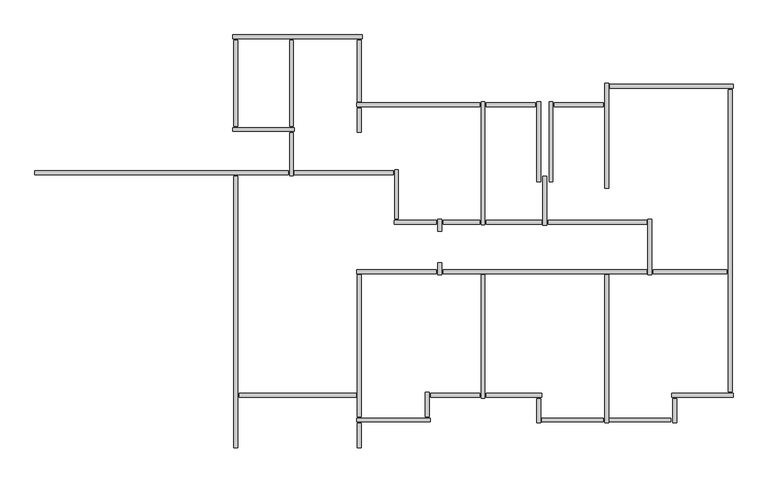
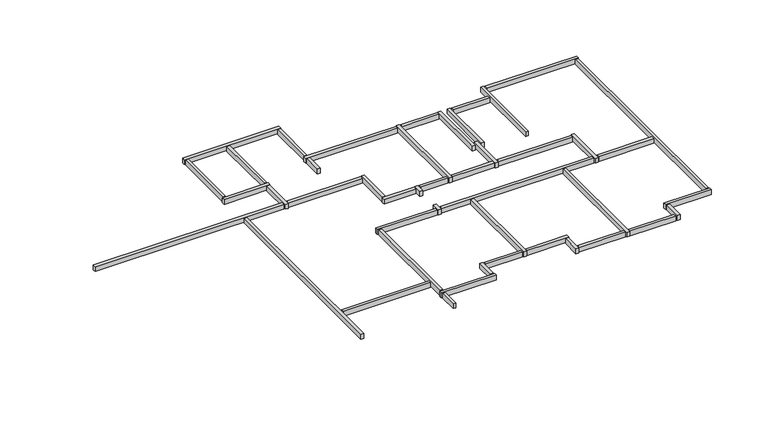
"""IFC4 building model written with IfcOpenShell, lengths in millimetres: beam geometry, Graute viga de respaldo12 : Graute viga de respaldo."""

from ifc_helpers import new_model, si_unit, frame, origin, place, context, project, spatial, polyline, outline, extrude, source, transform, mapped, element, save


def beam_e93206ce(model_context):
    return source(origin(), model_context, "Body", "SweptSolid", [
        extrude(outline(polyline([(-54994.9587292, 57408.4278788), (-54994.9587292, 57502.4278788), (-53804.9587292, 57502.4278788), (-53804.9587292, 57408.4278788), (-54994.9587292, 57408.4278788)])), frame((0.0, 0.0, 11632.9999999), z_axis=(0.0, 0.0, 1.0), x_axis=(1.0, 0.0, 0.0)), (0.0, 0.0, 1.0), 167.0),
        extrude(outline(polyline([(-56644.9587292, 57408.4278788), (-56644.9587292, 57502.4278788), (-55454.9587292, 57502.4278788), (-55454.9587292, 57408.4278788), (-56644.9587292, 57408.4278788)])), frame((0.0, 0.0, 11632.9999999), z_axis=(0.0, 0.0, 1.0), x_axis=(1.0, 0.0, 0.0)), (0.0, 0.0, 1.0), 167.0),
        extrude(outline(polyline([(-52594.9587292, 53358.4278788), (-52594.9587292, 53452.4278788), (-50804.9587292, 53452.4278788), (-50804.9587292, 53358.4278788), (-52594.9587292, 53358.4278788)])), frame((0.0, 0.0, 11632.9999999), z_axis=(0.0, 0.0, 1.0), x_axis=(1.0, 0.0, 0.0)), (0.0, 0.0, 1.0), 167.0),
        extrude(outline(polyline([(-57994.9587292, 50358.4278788), (-57994.9587292, 50452.4278788), (-56804.9587292, 50452.4278788), (-56804.9587292, 50358.4278788), (-57994.9587292, 50358.4278788)])), frame((0.0, 0.0, 11632.9999999), z_axis=(0.0, 0.0, 1.0), x_axis=(1.0, 0.0, 0.0)), (0.0, 0.0, 1.0), 167.0),
        extrude(outline(polyline([(-58121.9587292, 50475.4278788), (-58027.9587292, 50475.4278788), (-58027.9587292, 49885.4278788), (-58121.9587292, 49885.4278788), (-58121.9587292, 50475.4278788)])), frame((0.0, 0.0, 11632.9999999), z_axis=(0.0, 0.0, 1.0), x_axis=(1.0, 0.0, 0.0)), (0.0, 0.0, 1.0), 167.0),
        extrude(outline(polyline([(-59794.9587292, 49758.4278788), (-59794.9587292, 49852.4278788), (-58004.9587292, 49852.4278788), (-58004.9587292, 49758.4278788), (-59794.9587292, 49758.4278788)])), frame((0.0, 0.0, 11632.9999999), z_axis=(0.0, 0.0, 1.0), x_axis=(1.0, 0.0, 0.0)), (0.0, 0.0, 1.0), 167.0),
        extrude(outline(polyline([(-57727.9587292, 53335.4278788), (-57821.9587292, 53335.4278788), (-57821.9587292, 53625.4278788), (-57727.9587292, 53625.4278788), (-57727.9587292, 53335.4278788)])), frame((0.0, 0.0, 11632.9999999), z_axis=(0.0, 0.0, 1.0), x_axis=(1.0, 0.0, 0.0)), (0.0, 0.0, 1.0), 167.0),
        extrude(outline(polyline([(-55144.9587292, 54558.4278788), (-55144.9587292, 54652.4278788), (-52754.9587292, 54652.4278788), (-52754.9587292, 54558.4278788), (-55144.9587292, 54558.4278788)])), frame((0.0, 0.0, 11632.9999999), z_axis=(0.0, 0.0, 1.0), x_axis=(1.0, 0.0, 0.0)), (0.0, 0.0, 1.0), 167.0),
        extrude(outline(polyline([(-56644.9587292, 54558.4278788), (-56644.9587292, 54652.4278788), (-55304.9587292, 54652.4278788), (-55304.9587292, 54558.4278788), (-56644.9587292, 54558.4278788)])), frame((0.0, 0.0, 11632.9999999), z_axis=(0.0, 0.0, 1.0), x_axis=(1.0, 0.0, 0.0)), (0.0, 0.0, 1.0), 167.0),
        extrude(outline(polyline([(-57694.9587292, 54558.4278788), (-57694.9587292, 54652.4278788), (-56804.9587292, 54652.4278788), (-56804.9587292, 54558.4278788), (-57694.9587292, 54558.4278788)])), frame((0.0, 0.0, 11632.9999999), z_axis=(0.0, 0.0, 1.0), x_axis=(1.0, 0.0, 0.0)), (0.0, 0.0, 1.0), 167.0),
        extrude(outline(polyline([(-57727.9587292, 54385.4278788), (-57821.9587292, 54385.4278788), (-57821.9587292, 54675.4278788), (-57727.9587292, 54675.4278788), (-57727.9587292, 54385.4278788)])), frame((0.0, 0.0, 11632.9999999), z_axis=(0.0, 0.0, 1.0), x_axis=(1.0, 0.0, 0.0)), (0.0, 0.0, 1.0), 167.0),
        extrude(outline(polyline([(-58884.9587292, 54558.4278788), (-58884.9587292, 54652.4278788), (-57854.9587292, 54652.4278788), (-57854.9587292, 54558.4278788), (-58884.9587292, 54558.4278788)])), frame((0.0, 0.0, 11632.9999999), z_axis=(0.0, 0.0, 1.0), x_axis=(1.0, 0.0, 0.0)), (0.0, 0.0, 1.0), 167.0),
        extrude(outline(polyline([(-58871.9587292, 55875.4278788), (-58777.9587292, 55875.4278788), (-58777.9587292, 54685.4278788), (-58871.9587292, 54685.4278788), (-58871.9587292, 55875.4278788)])), frame((0.0, 0.0, 11632.9999999), z_axis=(0.0, 0.0, 1.0), x_axis=(1.0, 0.0, 0.0)), (0.0, 0.0, 1.0), 167.0),
        extrude(outline(polyline([(-61304.9587292, 55758.4278788), (-61304.9587292, 55852.4278788), (-58904.9587292, 55852.4278788), (-58904.9587292, 55758.4278788), (-61304.9587292, 55758.4278788)])), frame((0.0, 0.0, 11632.9999999), z_axis=(0.0, 0.0, 1.0), x_axis=(1.0, 0.0, 0.0)), (0.0, 0.0, 1.0), 167.0),
        extrude(outline(polyline([(-56677.9587292, 54540.4278788), (-56771.9587292, 54540.4278788), (-56771.9587292, 57525.4278788), (-56677.9587292, 57525.4278788), (-56677.9587292, 54540.4278788)])), frame((0.0, 0.0, 11632.9999999), z_axis=(0.0, 0.0, 1.0), x_axis=(1.0, 0.0, 0.0)), (0.0, 0.0, 1.0), 167.0),
        extrude(outline(polyline([(-59794.9587292, 57408.4278788), (-59794.9587292, 57502.4278788), (-56804.9587292, 57502.4278788), (-56804.9587292, 57408.4278788), (-59794.9587292, 57408.4278788)])), frame((0.0, 0.0, 11632.9999999), z_axis=(0.0, 0.0, 1.0), x_axis=(1.0, 0.0, 0.0)), (0.0, 0.0, 1.0), 167.0),
        extrude(outline(polyline([(-59677.9587292, 56785.4278788), (-59771.9587292, 56785.4278788), (-59771.9587292, 57375.4278788), (-59677.9587292, 57375.4278788), (-59677.9587292, 56785.4278788)])), frame((0.0, 0.0, 11632.9999999), z_axis=(0.0, 0.0, 1.0), x_axis=(1.0, 0.0, 0.0)), (0.0, 0.0, 1.0), 167.0),
        extrude(outline(polyline([(-59771.9587292, 59025.4278788), (-59677.9587292, 59025.4278788), (-59677.9587292, 57535.4278788), (-59771.9587292, 57535.4278788), (-59771.9587292, 59025.4278788)])), frame((0.0, 0.0, 11632.9999999), z_axis=(0.0, 0.0, 1.0), x_axis=(1.0, 0.0, 0.0)), (0.0, 0.0, 1.0), 167.0),
        extrude(outline(polyline([(-62771.9587292, 59025.4278788), (-62677.9587292, 59025.4278788), (-62677.9587292, 56935.4278788), (-62771.9587292, 56935.4278788), (-62771.9587292, 59025.4278788)])), frame((0.0, 0.0, 11632.9999999), z_axis=(0.0, 0.0, 1.0), x_axis=(1.0, 0.0, 0.0)), (0.0, 0.0, 1.0), 167.0),
        extrude(outline(polyline([(-61421.9587292, 59025.4278788), (-61327.9587292, 59025.4278788), (-61327.9587292, 56935.4278788), (-61421.9587292, 56935.4278788), (-61421.9587292, 59025.4278788)])), frame((0.0, 0.0, 11632.9999999), z_axis=(0.0, 0.0, 1.0), x_axis=(1.0, 0.0, 0.0)), (0.0, 0.0, 1.0), 167.0),
        extrude(outline(polyline([(-61327.9587292, 55735.4278788), (-61421.9587292, 55735.4278788), (-61421.9587292, 56775.4278788), (-61327.9587292, 56775.4278788), (-61327.9587292, 55735.4278788)])), frame((0.0, 0.0, 11632.9999999), z_axis=(0.0, 0.0, 1.0), x_axis=(1.0, 0.0, 0.0)), (0.0, 0.0, 1.0), 167.0),
        extrude(outline(polyline([(-62644.9587292, 50358.4278788), (-62644.9587292, 50452.4278788), (-59804.9587292, 50452.4278788), (-59804.9587292, 50358.4278788), (-62644.9587292, 50358.4278788)])), frame((0.0, 0.0, 11632.9999999), z_axis=(0.0, 0.0, 1.0), x_axis=(1.0, 0.0, 0.0)), (0.0, 0.0, 1.0), 167.0),
        extrude(outline(polyline([(-59771.9587292, 53325.4278788), (-59677.9587292, 53325.4278788), (-59677.9587292, 49885.4278788), (-59771.9587292, 49885.4278788), (-59771.9587292, 53325.4278788)])), frame((0.0, 0.0, 11632.9999999), z_axis=(0.0, 0.0, 1.0), x_axis=(1.0, 0.0, 0.0)), (0.0, 0.0, 1.0), 167.0),
        extrude(outline(polyline([(-59794.9587292, 53358.4278788), (-59794.9587292, 53452.4278788), (-57854.9587292, 53452.4278788), (-57854.9587292, 53358.4278788), (-59794.9587292, 53358.4278788)])), frame((0.0, 0.0, 11632.9999999), z_axis=(0.0, 0.0, 1.0), x_axis=(1.0, 0.0, 0.0)), (0.0, 0.0, 1.0), 167.0),
        extrude(outline(polyline([(-57694.9587292, 53358.4278788), (-57694.9587292, 53452.4278788), (-52754.9587292, 53452.4278788), (-52754.9587292, 53358.4278788), (-57694.9587292, 53358.4278788)])), frame((0.0, 0.0, 11632.9999999), z_axis=(0.0, 0.0, 1.0), x_axis=(1.0, 0.0, 0.0)), (0.0, 0.0, 1.0), 167.0),
        extrude(outline(polyline([(-56677.9587292, 50335.4278788), (-56771.9587292, 50335.4278788), (-56771.9587292, 53325.4278788), (-56677.9587292, 53325.4278788), (-56677.9587292, 50335.4278788)])), frame((0.0, 0.0, 11632.9999999), z_axis=(0.0, 0.0, 1.0), x_axis=(1.0, 0.0, 0.0)), (0.0, 0.0, 1.0), 167.0),
        extrude(outline(polyline([(-55304.9587292, 50452.4278788), (-55304.9587292, 50358.4278788), (-56644.9587292, 50358.4278788), (-56644.9587292, 50452.4278788), (-55304.9587292, 50452.4278788)])), frame((0.0, 0.0, 11632.9999999), z_axis=(0.0, 0.0, 1.0), x_axis=(1.0, 0.0, 0.0)), (0.0, 0.0, 1.0), 167.0),
        extrude(outline(polyline([(-55327.9587292, 49735.4278788), (-55421.9587292, 49735.4278788), (-55421.9587292, 50325.4278788), (-55327.9587292, 50325.4278788), (-55327.9587292, 49735.4278788)])), frame((0.0, 0.0, 11632.9999999), z_axis=(0.0, 0.0, 1.0), x_axis=(1.0, 0.0, 0.0)), (0.0, 0.0, 1.0), 167.0),
        extrude(outline(polyline([(-55294.9587292, 49758.4278788), (-55294.9587292, 49852.4278788), (-53804.9587292, 49852.4278788), (-53804.9587292, 49758.4278788), (-55294.9587292, 49758.4278788)])), frame((0.0, 0.0, 11632.9999999), z_axis=(0.0, 0.0, 1.0), x_axis=(1.0, 0.0, 0.0)), (0.0, 0.0, 1.0), 167.0),
        extrude(outline(polyline([(-52165.9809043, 49853.4278788), (-52165.9809043, 49758.4278788), (-53654.9587292, 49758.4278788), (-53654.9587292, 49853.4278788), (-52165.9809043, 49853.4278788)])), frame((0.0, 0.0, 11617.1856208), z_axis=(0.0, 0.0, 1.0), x_axis=(1.0, 0.0, 0.0)), (0.0, 0.0, 1.0), 165.0),
        extrude(outline(polyline([(-50771.9587292, 57825.4278788), (-50677.9587292, 57825.4278788), (-50677.9587292, 50485.4278788), (-50771.9587292, 50485.4278788), (-50771.9587292, 57825.4278788)])), frame((0.0, 0.0, 11632.9999999), z_axis=(0.0, 0.0, 1.0), x_axis=(1.0, 0.0, 0.0)), (0.0, 0.0, 1.0), 167.0),
        extrude(outline(polyline([(-52721.9587292, 54675.4278788), (-52627.9587292, 54675.4278788), (-52627.9587292, 53330.0746661), (-52721.9587292, 53330.0746661), (-52721.9587292, 54675.4278788)])), frame((0.0, 0.0, 11632.9999999), z_axis=(0.0, 0.0, 1.0), x_axis=(1.0, 0.0, 0.0)), (0.0, 0.0, 1.0), 167.0),
        extrude(outline(polyline([(-55271.9587292, 55725.4278788), (-55177.9587292, 55725.4278788), (-55177.9587292, 54535.4278788), (-55271.9587292, 54535.4278788), (-55271.9587292, 55725.4278788)])), frame((0.0, 0.0, 11632.9999999), z_axis=(0.0, 0.0, 1.0), x_axis=(1.0, 0.0, 0.0)), (0.0, 0.0, 1.0), 167.0),
        extrude(outline(polyline([(-55121.9587292, 57525.4278788), (-55027.9587292, 57525.4278788), (-55027.9587292, 55585.4278788), (-55121.9587292, 55585.4278788), (-55121.9587292, 57525.4278788)])), frame((0.0, 0.0, 11632.9999999), z_axis=(0.0, 0.0, 1.0), x_axis=(1.0, 0.0, 0.0)), (0.0, 0.0, 1.0), 167.0),
        extrude(outline(polyline([(-55421.9587292, 57525.4278788), (-55327.9587292, 57525.4278788), (-55327.9587292, 55585.4278788), (-55421.9587292, 55585.4278788), (-55421.9587292, 57525.4278788)])), frame((0.0, 0.0, 11632.9999999), z_axis=(0.0, 0.0, 1.0), x_axis=(1.0, 0.0, 0.0)), (0.0, 0.0, 1.0), 167.0),
        extrude(outline(polyline([(-53771.9587292, 57975.4278788), (-53677.9587292, 57975.4278788), (-53677.9587292, 55435.4278788), (-53771.9587292, 55435.4278788), (-53771.9587292, 57975.4278788)])), frame((0.0, 0.0, 11632.9999999), z_axis=(0.0, 0.0, 1.0), x_axis=(1.0, 0.0, 0.0)), (0.0, 0.0, 1.0), 167.0),
        extrude(outline(polyline([(-50654.9587292, 57952.4278788), (-50654.9587292, 57858.4278788), (-53644.9587292, 57858.4278788), (-53644.9587292, 57952.4278788), (-50654.9587292, 57952.4278788)])), frame((0.0, 0.0, 11632.9999999), z_axis=(0.0, 0.0, 1.0), x_axis=(1.0, 0.0, 0.0)), (0.0, 0.0, 1.0), 167.0),
        extrude(outline(polyline([(-52027.9587292, 49735.4278788), (-52121.9587292, 49735.4278788), (-52121.9587292, 50325.4278788), (-52027.9587292, 50325.4278788), (-52027.9587292, 49735.4278788)])), frame((0.0, 0.0, 11632.9999999), z_axis=(0.0, 0.0, 1.0), x_axis=(1.0, 0.0, 0.0)), (0.0, 0.0, 1.0), 167.0),
        extrude(outline(polyline([(-52144.9587292, 50358.4278788), (-52144.9587292, 50452.4278788), (-50654.9587292, 50452.4278788), (-50654.9587292, 50358.4278788), (-52144.9587292, 50358.4278788)])), frame((0.0, 0.0, 11632.9999999), z_axis=(0.0, 0.0, 1.0), x_axis=(1.0, 0.0, 0.0)), (0.0, 0.0, 1.0), 167.0),
        extrude(outline(polyline([(-53677.9587292, 49735.4278788), (-53771.9587292, 49735.4278788), (-53771.9587292, 53325.4278788), (-53677.9587292, 53325.4278788), (-53677.9587292, 49735.4278788)])), frame((0.0, 0.0, 11632.9999999), z_axis=(0.0, 0.0, 1.0), x_axis=(1.0, 0.0, 0.0)), (0.0, 0.0, 1.0), 167.0),
        extrude(outline(polyline([(-59677.9587292, 49135.4278788), (-59771.9587292, 49135.4278788), (-59771.9587292, 49725.4278788), (-59677.9587292, 49725.4278788), (-59677.9587292, 49135.4278788)])), frame((0.0, 0.0, 11632.9999999), z_axis=(0.0, 0.0, 1.0), x_axis=(1.0, 0.0, 0.0)), (0.0, 0.0, 1.0), 167.0),
        extrude(outline(polyline([(-62794.9587292, 56808.4278788), (-62794.9587292, 56902.4278788), (-61304.9587292, 56902.4278788), (-61304.9587292, 56808.4278788), (-62794.9587292, 56808.4278788)])), frame((0.0, 0.0, 11632.9999999), z_axis=(0.0, 0.0, 1.0), x_axis=(1.0, 0.0, 0.0)), (0.0, 0.0, 1.0), 167.0),
        extrude(outline(polyline([(-62794.9587292, 59058.4278788), (-62794.9587292, 59152.4278788), (-59654.9587292, 59152.4278788), (-59654.9587292, 59058.4278788), (-62794.9587292, 59058.4278788)])), frame((0.0, 0.0, 11632.9999999), z_axis=(0.0, 0.0, 1.0), x_axis=(1.0, 0.0, 0.0)), (0.0, 0.0, 1.0), 167.0),
        extrude(outline(polyline([(-67601.7587292, 55758.4278788), (-67601.7587292, 55852.4278788), (-61454.9587292, 55852.4278788), (-61454.9587292, 55758.4278788), (-67601.7587292, 55758.4278788)])), frame((0.0, 0.0, 11632.9999999), z_axis=(0.0, 0.0, 1.0), x_axis=(1.0, 0.0, 0.0)), (0.0, 0.0, 1.0), 167.0),
        extrude(outline(polyline([(-62677.9587292, 49132.8979841), (-62771.9587292, 49132.8979841), (-62771.9587292, 55725.4278788), (-62677.9587292, 55725.4278788), (-62677.9587292, 49132.8979841)])), frame((0.0, 0.0, 11632.9999999), z_axis=(0.0, 0.0, 1.0), x_axis=(1.0, 0.0, 0.0)), (0.0, 0.0, 1.0), 167.0),
    ])


if __name__ == "__main__":
    model = new_model("IFC4")
    model_context = context("Model", 3, world=origin())
    ifc_project = project(units=[si_unit("LENGTHUNIT", "METRE", prefix="MILLI")], contexts=[model_context])
    site = spatial("IfcSite", under=ifc_project)
    building = spatial("IfcBuilding", under=site)
    placement = place(None, origin())
    beam_shape = beam_e93206ce(model_context)
    element("IfcBeam", 1, ObjectType="Graute viga de respaldo12 : Graute viga de respaldo", at=placement, inside=building, context=model_context, shape_type="MappedRepresentation", body=[
        mapped(beam_shape, transform((0.0, 0.0, 0.0), x_axis=(1.0, 0.0, 0.0), y_axis=(0.0, 1.0, 0.0), z_axis=(0.0, 0.0, 1.0))),
    ])
    save(model, "model.ifc")

# Revit data of these elements
# Element 1 (IfcBeam, "Graute viga de respaldo12 : Graute viga de respaldo")
#   Materials on its faces: "Concreto, Faixa de areia/cimento"
# Materials
#   "Concreto, Faixa de areia/cimento": class "Concreto", colour RGB 127 127 127, transparency 0, Description = "Revestimento de laje de concreto", Cost = 0
